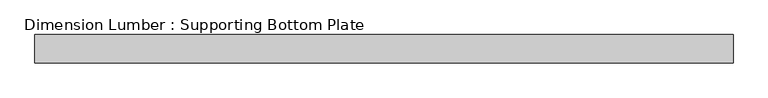
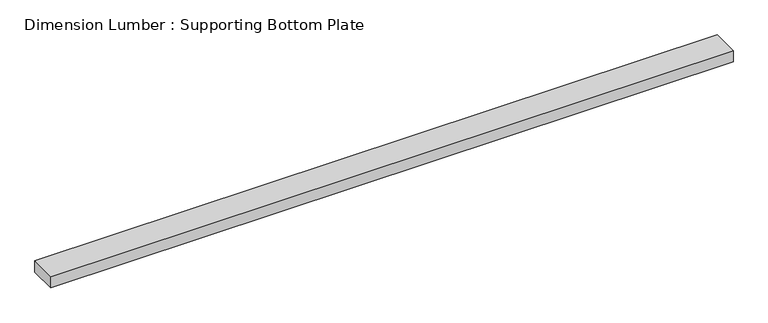
"""IFC4 building model written with IfcOpenShell, lengths in millimetres: beam geometry, Dimension Lumber : Supporting Bottom Plate."""

from ifc_helpers import new_model, si_unit, frame, origin, place, context, project, spatial, polyline, outline, extrude, source, transform, mapped, element, save


def dimension_lumber_supporting_bottom_plate_d1710e57(model_context):
    return source(origin(), model_context, "Body", "SweptSolid", [
        extrude(outline(polyline([(1739.2219145, 44.45), (1739.2219145, -44.45), (-454.81875, -44.45), (-454.81875, 44.45), (1739.2219145, 44.45)])), frame((0.0, 0.0, -19.05), z_axis=(0.0, 0.0, 1.0), x_axis=(1.0, 0.0, 0.0)), (0.0, 0.0, 1.0), 38.1),
    ])


if __name__ == "__main__":
    model = new_model("IFC4")
    model_context = context("Model", 3, world=origin())
    ifc_project = project(units=[si_unit("LENGTHUNIT", "METRE", prefix="MILLI")], contexts=[model_context])
    site = spatial("IfcSite", under=ifc_project)
    building = spatial("IfcBuilding", under=site)
    placement = place(None, origin())
    dimension_lumber_supporting_bottom_plate_shape = dimension_lumber_supporting_bottom_plate_d1710e57(model_context)
    element("IfcBeam", 1, ObjectType="Dimension Lumber : Supporting Bottom Plate", at=placement, inside=building, context=model_context, shape_type="MappedRepresentation", body=[
        mapped(dimension_lumber_supporting_bottom_plate_shape, transform((0.0, 0.0, 0.0), x_axis=(1.0, 0.0, 0.0), y_axis=(0.0, 1.0, 0.0), z_axis=(0.0, 0.0, 1.0))),
    ])
    save(model, "model.ifc")

# Revit data of these elements
# Type "Dimension Lumber : Supporting Bottom Plate"
#   Assembly Code = "B10"
#   A = 0.0364583 SF
#   Length [instance default] = 5' - 0"
#   b = 0' - 3 1/2"
#   d = 0' - 1 1/2"
#   Structural Material [instance default] = Softwood, Lumber
# Element 1 (IfcBeam, "Dimension Lumber : Supporting Bottom Plate")
#   Structural Material = Douglas Fir #2
#   Materials on its faces: "Douglas Fir #2"
# Materials
#   "Softwood, Lumber": class "Wood", colour RGB 223 192 134, transparency 0, Description = "Pinus Echinata", Cost = 0
#   "Douglas Fir #2": class "Wood", colour RGB 223 192 134, transparency 0, Description = "Pinus Echinata", Cost = 0
